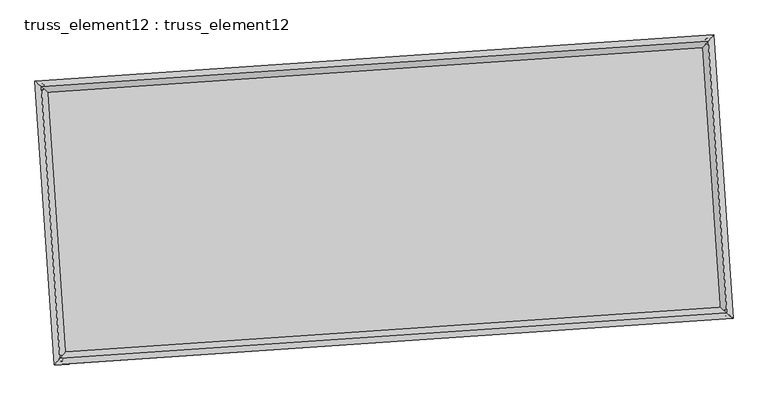
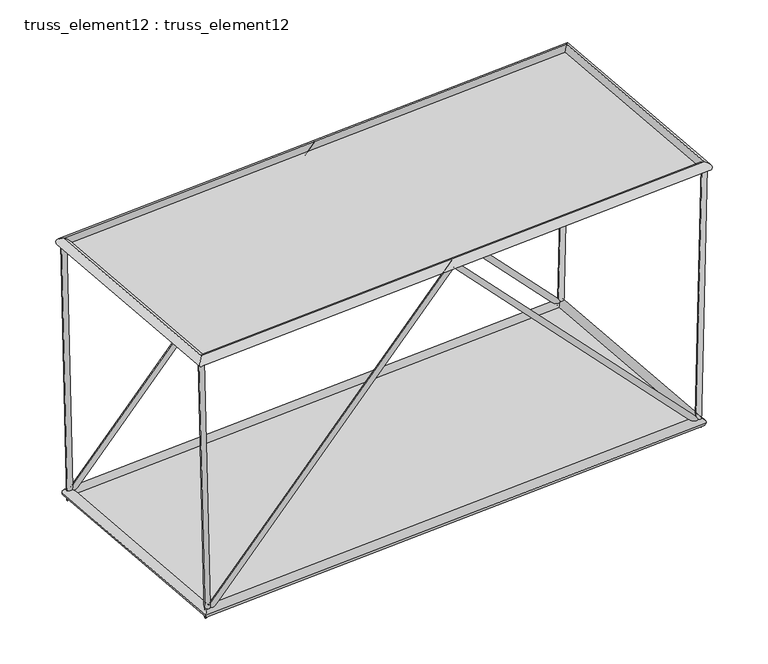
"""IFC4 building model written with IfcOpenShell, lengths in millimetres: plate geometry, truss_element12 : truss_element12."""

from ifc_helpers import new_model, si_unit, frame, origin, origin_with_axes, place, context, project, spatial, polyline, circle_curve, ellipse_curve, outline, extrude, source, transform, mapped, element, save
from ifc_brep_helpers import plane_surface, cylinder_surface, advanced_brep


def truss_element12_truss_element12_13b70bee(model_context):
    return source(origin(), model_context, "Body", "SolidModel", [
        advanced_brep(
        [(-3781.3878429, 2268.2839414, 4999.8023514), (-3880.4640895, 2254.9245561, 4997.4733651), (-3667.7523744, 2276.0323121, 121.2466732), (-3761.2345085, 2263.054368, -121.2466732), (1063.5274158, 2598.6402957, 5070.7560552), (1063.9784835, 2592.0672996, 4926.528566), (5795.1821195, 2921.2738432, 121.2492756), (5889.5788575, 2921.1066453, -121.2492756), (5908.4454526, 2928.9968394, 4999.8074441), (6008.4182784, 2929.2098536, 4997.4860818)],
        [
            (0, 1, circle_curve(frame((-3830.9259662, 2261.6042488, 4998.6378583), z_axis=(-0.02328650495741506, -0.0015878182527536, 0.9997275716514298), x_axis=(-0.13359443840271754, 0.9910348940631258, -0.001537783193974795)), 50.0)),
            (1, 0, circle_curve(frame((-3830.9259662, 2261.6042488, 4998.6378583), z_axis=(-0.02328650495741506, -0.0015878182527536, 0.9997275716514298), x_axis=(-0.13359443840271754, 0.9910348940631258, -0.001537783193974795)), 50.0)),
            (0, 2),
            (2, 3, ellipse_curve(frame((-3714.4934414, 2269.54334, 0.0), z_axis=(-0.9300456480783869, -0.06341627730797174, 0.36193019805323257), x_axis=(0.36109174913580183, 0.024621473735326325, 0.9322051982997884)), 130.347573, 50.0)),
            (3, 1),
            (3, 2, ellipse_curve(frame((-3714.4934414, 2269.54334, 0.0), z_axis=(-0.9300456480783869, -0.06341627730797174, 0.36193019805323257), x_axis=(0.36109174913580183, 0.024621473735326325, 0.9322051982997884)), 130.347573, 50.0)),
            (2, 4),
            (4, 5, ellipse_curve(frame((1063.7529497, 2595.3537976, 4998.6423106), z_axis=(-0.9976833958768767, -0.06802823821520047, -1.992283297939691e-05), x_axis=(1.9876679666230083e-05, 1.3553152281842393e-06, -0.9999999998015403)), 72.2707708, 50.0)),
            (5, 3),
            (5, 4, ellipse_curve(frame((1063.7529497, 2595.3537976, 4998.6423106), z_axis=(-0.9976833958768767, -0.06802823821520047, -1.992283297939691e-05), x_axis=(1.9876679666230083e-05, 1.3553152281842393e-06, -0.9999999998015403)), 72.2707708, 50.0)),
            (4, 6),
            (6, 7, ellipse_curve(frame((5842.3804885, 2921.1902443, 0.0), z_axis=(-0.9300246539008387, -0.06341484579481112, -0.3619843925771465), x_axis=(-0.3611458181124689, -0.024625160493309917, 0.9321841553741161)), 130.3533132, 50.0)),
            (7, 5),
            (7, 6, ellipse_curve(frame((5842.3804885, 2921.1902443, 0.0), z_axis=(-0.9300246539008387, -0.06341484579481112, -0.3619843925771465), x_axis=(-0.3611458181124689, -0.024625160493309917, 0.9321841553741161)), 130.3533132, 50.0)),
            (8, 9, circle_curve(frame((5958.4318655, 2929.1033465, 4998.6467629), z_axis=(0.023210275405573154, 0.0015826204493890937, 0.9997293525890448), x_axis=(-0.0021663046918160016, 0.9999964788957632, -0.0015327491829060865)), 50.0)),
            (9, 8, circle_curve(frame((5958.4318655, 2929.1033465, 4998.6467629), z_axis=(0.023210275405573154, 0.0015826204493890937, 0.9997293525890448), x_axis=(-0.0021663046918160016, 0.9999964788957632, -0.0015327491829060865)), 50.0)),
            (6, 8),
            (9, 7),
        ],
        [
            plane_surface(frame((-3830.9259662, 2311.6041857, 4998.7172707), z_axis=(-0.023286504957416205, -0.0015878182527521672, 0.9997275716514298), x_axis=(0.9997288325775486, -3.698476667768344e-05, 0.023286475586889552))),
            cylinder_surface(frame((-3830.9259662, 2261.6042488, 4998.6378583), z_axis=(-0.02328650495741506, -0.0015878182527536, 0.9997275716514298), x_axis=(-0.13359443840271754, 0.9910348940631258, -0.001537783193974795)), 50.0),
            cylinder_surface(frame((-3714.4934414, 2269.54334, 0.0), z_axis=(-0.6902255509886958, -0.047063856528962014, -0.7220621040956053), x_axis=(-0.02041790482368491, 0.9987519716635986, -0.045580788285038025)), 50.0),
            cylinder_surface(frame((1063.7529497, 2595.3537976, 4998.6423106), z_axis=(-0.690254254835047, -0.04706581373513127, 0.7220345371653382), x_axis=(-0.11534114330815694, 0.9922795168683531, -0.045582683816059205)), 50.0),
            plane_surface(frame((5958.4318655, 2879.1034091, 4998.7259153), z_axis=(0.023210275405573518, 0.0015826204493892728, 0.9997293525890449), x_axis=(0.9997306052710389, -3.674295485112107e-05, -0.023210246322644654))),
            cylinder_surface(frame((5842.3804885, 2921.1902443, 0.0), z_axis=(-0.023210275405573154, -0.0015826204493890937, -0.9997293525890448), x_axis=(-0.0021663046918160016, 0.9999964788957632, -0.0015327491829060865)), 50.0),
        ],
        [
            (0, [[1, 2]]),
            (1, [[-1, 3, 4, 5]]),
            (1, [[-2, -5, 6, -3]]),
            (2, [[-4, 7, 8, 9]]),
            (2, [[-6, -9, 10, -7]]),
            (3, [[-8, 11, 12, 13]]),
            (3, [[-10, -13, 14, -11]]),
            (4, [[15, 16]]),
            (5, [[-12, 17, -16, 18]]),
            (5, [[-14, -18, -15, -17]]),
        ],
    ),
        advanced_brep(
        [(-3509.27489, -1722.4496429, 4999.8023514), (-3608.3511366, -1735.8090282, 4997.4733651), (-3395.6394215, -1714.7012722, 121.2466732), (-3489.1215555, -1727.6792163, -121.2466732), (1335.6403687, -1392.0932886, 5070.7560552), (1336.0914364, -1398.6662847, 4926.528566), (6067.2950724, -1069.4597411, 121.2492756), (6161.6918104, -1069.626939, -121.2492756), (6180.5584055, -1061.7367449, 4999.8074441), (6280.5312314, -1061.5237307, 4997.4860818)],
        [
            (0, 1, circle_curve(frame((-3558.8130133, -1729.1293355, 4998.6378583), z_axis=(-0.023286504957415285, -0.0015878182527535897, 0.9997275716514298), x_axis=(-0.13359443840271787, 0.9910348940631256, -0.0015377831939748436)), 50.0)),
            (1, 0, circle_curve(frame((-3558.8130133, -1729.1293355, 4998.6378583), z_axis=(-0.023286504957415285, -0.0015878182527535897, 0.9997275716514298), x_axis=(-0.13359443840271787, 0.9910348940631256, -0.0015377831939748436)), 50.0)),
            (0, 2),
            (2, 3, ellipse_curve(frame((-3442.3804885, -1721.1902443, 0.0), z_axis=(-0.9300456480783867, -0.06341627730797184, 0.3619301980532322), x_axis=(0.3610917491358014, 0.024621473735326367, 0.9322051982997887)), 130.347573, 50.0)),
            (3, 1),
            (3, 2, ellipse_curve(frame((-3442.3804885, -1721.1902443, 0.0), z_axis=(-0.9300456480783867, -0.06341627730797184, 0.3619301980532322), x_axis=(0.3610917491358014, 0.024621473735326367, 0.9322051982997887)), 130.347573, 50.0)),
            (2, 4),
            (4, 5, ellipse_curve(frame((1335.8659026, -1395.3797867, 4998.6423106), z_axis=(-0.9976833958768767, -0.06802823821520053, -1.9922832979958566e-05), x_axis=(1.9876679666998888e-05, 1.3553152281361895e-06, -0.9999999998015403)), 72.2707708, 50.0)),
            (5, 3),
            (5, 4, ellipse_curve(frame((1335.8659026, -1395.3797867, 4998.6423106), z_axis=(-0.9976833958768767, -0.06802823821520053, -1.9922832979958566e-05), x_axis=(1.9876679666998888e-05, 1.3553152281361895e-06, -0.9999999998015403)), 72.2707708, 50.0)),
            (4, 6),
            (6, 7, ellipse_curve(frame((6114.4934414, -1069.54334, 0.0), z_axis=(-0.9300246539008382, -0.06341484579481105, -0.3619843925771475), x_axis=(-0.3611458181124699, -0.02462516049330997, 0.9321841553741157)), 130.3533132, 50.0)),
            (7, 5),
            (7, 6, ellipse_curve(frame((6114.4934414, -1069.54334, 0.0), z_axis=(-0.9300246539008382, -0.06341484579481105, -0.3619843925771475), x_axis=(-0.3611458181124699, -0.02462516049330997, 0.9321841553741157)), 130.3533132, 50.0)),
            (8, 9, circle_curve(frame((6230.5448184, -1061.6302378, 4998.6467629), z_axis=(0.023210275405571995, 0.0015826204493890016, 0.9997293525890449), x_axis=(-0.002166304691815724, 0.9999964788957632, -0.001532749182906003)), 50.0)),
            (9, 8, circle_curve(frame((6230.5448184, -1061.6302378, 4998.6467629), z_axis=(0.023210275405571995, 0.0015826204493890016, 0.9997293525890449), x_axis=(-0.002166304691815724, 0.9999964788957632, -0.001532749182906003)), 50.0)),
            (6, 8),
            (9, 7),
        ],
        [
            plane_surface(frame((-3558.8130133, -1679.1293986, 4998.7172707), z_axis=(-0.023286504957416205, -0.0015878182527521672, 0.9997275716514298), x_axis=(0.9997288325775486, -3.698476667768344e-05, 0.023286475586889552))),
            cylinder_surface(frame((-3558.8130133, -1729.1293355, 4998.6378583), z_axis=(-0.023286504957415282, -0.0015878182527535893, 0.9997275716514296), x_axis=(-0.13359443840271787, 0.9910348940631256, -0.0015377831939748436)), 50.0),
            cylinder_surface(frame((-3442.3804885, -1721.1902443, 0.0), z_axis=(-0.6902255509886953, -0.0470638565289621, -0.7220621040956057), x_axis=(-0.020417904823684878, 0.9987519716635985, -0.04558078828503815)), 50.0),
            cylinder_surface(frame((1335.8659026, -1395.3797867, 4998.6423106), z_axis=(-0.6902542548350474, -0.04706581373513127, 0.7220345371653377), x_axis=(-0.11534114330815701, 0.9922795168683533, -0.04558268381605939)), 50.0),
            plane_surface(frame((6230.5448184, -1111.6301752, 4998.7259153), z_axis=(0.023210275405573518, 0.0015826204493892728, 0.9997293525890449), x_axis=(0.9997306052710389, -3.674295485112107e-05, -0.023210246322644654))),
            cylinder_surface(frame((6114.4934414, -1069.54334, 0.0), z_axis=(-0.02321027540557199, -0.0015826204493890011, -0.9997293525890447), x_axis=(-0.002166304691815724, 0.9999964788957632, -0.001532749182906003)), 50.0),
        ],
        [
            (0, [[1, 2]]),
            (1, [[-1, 3, 4, 5]]),
            (1, [[-2, -5, 6, -3]]),
            (2, [[-4, 7, 8, 9]]),
            (2, [[-6, -9, 10, -7]]),
            (3, [[-8, 11, 12, 13]]),
            (3, [[-10, -13, 14, -11]]),
            (4, [[15, 16]]),
            (5, [[-12, 17, -16, 18]]),
            (5, [[-14, -18, -15, -17]]),
        ],
    ),
        advanced_brep(
        [(-3558.810702, -1729.1267739, 4908.6378583), (-3558.8153245, -1729.1318972, 5088.6378582), (-3830.9286038, 2261.606473, 5088.6378582), (-3830.9233286, 2261.6020246, 4908.6378583), (5958.4340138, 2929.105897, 5088.6467629), (5958.4297173, 2929.100796, 4908.646763), (6230.5472931, -1061.6324731, 5088.6467629), (6230.5423438, -1061.6280025, 4908.646763)],
        [
            (0, 1, ellipse_curve(frame((-3558.8130133, -1729.1293355, 4998.6378583), z_axis=(-0.7535719234051663, 0.6573654662781019, -6.417150933687318e-07), x_axis=(-0.6573654662777916, -0.753571923405437, -6.417150933687713e-07)), 127.2792206, 90.0)),
            (1, 2),
            (2, 3, ellipse_curve(frame((-3830.9259662, 2261.6042488, 4998.6378583), z_axis=(-0.6573654662777915, -0.7535719234054372, -6.417150933688095e-07), x_axis=(0.7535719234051665, -0.6573654662781016, 6.417150933687701e-07)), 127.2792206, 90.0)),
            (3, 0),
            (1, 0, ellipse_curve(frame((-3558.8130133, -1729.1293355, 4998.6378583), z_axis=(-0.7535719234051663, 0.6573654662781019, -6.417150933687318e-07), x_axis=(-0.6573654662777916, -0.753571923405437, -6.417150933687713e-07)), 127.2792206, 90.0)),
            (3, 2, ellipse_curve(frame((-3830.9259662, 2261.6042488, 4998.6378583), z_axis=(-0.6573654662777915, -0.7535719234054372, -6.417150933688095e-07), x_axis=(0.7535719234051665, -0.6573654662781016, 6.417150933687701e-07)), 127.2792206, 90.0)),
            (2, 4),
            (4, 5, ellipse_curve(frame((5958.4318655, 2929.1033465, 4998.6467629), z_axis=(-0.7535719234051664, 0.6573654662781019, -6.41715093368808e-07), x_axis=(-0.6573654662777914, -0.7535719234054371, -6.417150933687716e-07)), 127.2792206, 90.0)),
            (5, 3),
            (5, 4, ellipse_curve(frame((5958.4318655, 2929.1033465, 4998.6467629), z_axis=(-0.7535719234051664, 0.6573654662781019, -6.41715093368808e-07), x_axis=(-0.6573654662777914, -0.7535719234054371, -6.417150933687716e-07)), 127.2792206, 90.0)),
            (4, 6),
            (6, 7, ellipse_curve(frame((6230.5448184, -1061.6302378, 4998.6467629), z_axis=(0.6573654662777916, 0.753571923405437, 6.417150933687335e-07), x_axis=(-0.7535719234051662, 0.657365466278102, -6.417150933687697e-07)), 127.2792206, 90.0)),
            (7, 5),
            (7, 6, ellipse_curve(frame((6230.5448184, -1061.6302378, 4998.6467629), z_axis=(0.6573654662777916, 0.753571923405437, 6.417150933687335e-07), x_axis=(-0.7535719234051662, 0.657365466278102, -6.417150933687697e-07)), 127.2792206, 90.0)),
            (6, 1),
            (0, 7),
        ],
        [
            cylinder_surface(frame((-3558.8130133, -1729.1293355, 4998.6378583), z_axis=(0.06802823822869986, -0.9976833960748767, 0.0), x_axis=(-0.997683395696052, -0.06802823820286925, -2.7557367220821507e-05)), 90.0),
            cylinder_surface(frame((-3830.9259662, 2261.6042488, 4998.6378583), z_axis=(-0.9976833960744659, -0.06802823822867164, -9.075221882216596e-07), x_axis=(-0.06802823818041304, 0.9976833957222375, -2.6649845032922138e-05)), 90.0),
            cylinder_surface(frame((5958.4318655, 2929.1033465, 4998.6467629), z_axis=(-0.06802823822869951, 0.9976833960748768, 0.0), x_axis=(0.9976833957443108, 0.06802823820615947, -2.5742322845022792e-05)), 90.0),
            cylinder_surface(frame((6230.5448184, -1061.6302378, 4998.6467629), z_axis=(0.997683396074466, 0.06802823822867146, 9.075221882216056e-07), x_axis=(0.06802823822867146, -0.997683395718947, -2.6649845032922155e-05)), 90.0),
        ],
        [
            (0, [[1, 2, 3, 4]]),
            (0, [[5, -4, 6, -2]]),
            (1, [[-3, 7, 8, 9]]),
            (1, [[-6, -9, 10, -7]]),
            (2, [[-8, 11, 12, 13]]),
            (2, [[-10, -13, 14, -11]]),
            (3, [[-12, 15, -1, 16]]),
            (3, [[-14, -16, -5, -15]]),
        ],
    ),
        advanced_brep(
        [(-3358.7115243, -1625.2761972, 0.0), (-3526.0494527, -1817.1042913, 0.0), (-3810.4074885, 2353.2123043, 0.0), (-3618.5793943, 2185.8743758, 0.0), (5926.0494527, 3017.1042913, 0.0), (5758.7115243, 2825.2761972, 0.0), (6210.4074885, -1153.2123043, 0.0), (6018.5793943, -985.8743758, 0.0)],
        [
            (0, 1, ellipse_curve(frame((-3442.3804885, -1721.1902443, 0.0), z_axis=(-0.7535719234054579, 0.6573654662780808, 0.0), x_axis=(-0.6573654662780808, -0.753571923405458, 0.0)), 127.2792206, 90.0)),
            (1, 2),
            (2, 3, ellipse_curve(frame((-3714.4934414, 2269.54334, 0.0), z_axis=(-0.6573654662780807, -0.7535719234054581, 0.0), x_axis=(0.7535719234054581, -0.6573654662780806, 0.0)), 127.2792206, 90.0)),
            (3, 0),
            (1, 0, ellipse_curve(frame((-3442.3804885, -1721.1902443, 0.0), z_axis=(-0.7535719234054579, 0.6573654662780808, 0.0), x_axis=(-0.6573654662780808, -0.753571923405458, 0.0)), 127.2792206, 90.0)),
            (3, 2, ellipse_curve(frame((-3714.4934414, 2269.54334, 0.0), z_axis=(-0.6573654662780807, -0.7535719234054581, 0.0), x_axis=(0.7535719234054581, -0.6573654662780806, 0.0)), 127.2792206, 90.0)),
            (2, 4),
            (4, 5, ellipse_curve(frame((5842.3804885, 2921.1902443, 0.0), z_axis=(-0.7535719234054578, 0.657365466278081, 0.0), x_axis=(-0.657365466278081, -0.7535719234054578, 0.0)), 127.2792206, 90.0)),
            (5, 3),
            (5, 4, ellipse_curve(frame((5842.3804885, 2921.1902443, 0.0), z_axis=(-0.7535719234054578, 0.657365466278081, 0.0), x_axis=(-0.657365466278081, -0.7535719234054578, 0.0)), 127.2792206, 90.0)),
            (4, 6),
            (6, 7, ellipse_curve(frame((6114.4934414, -1069.54334, 0.0), z_axis=(0.6573654662780811, 0.7535719234054576, 0.0), x_axis=(-0.7535719234054576, 0.6573654662780812, 0.0)), 127.2792206, 90.0)),
            (7, 5),
            (7, 6, ellipse_curve(frame((6114.4934414, -1069.54334, 0.0), z_axis=(0.6573654662780811, 0.7535719234054576, 0.0), x_axis=(-0.7535719234054576, 0.6573654662780812, 0.0)), 127.2792206, 90.0)),
            (6, 1),
            (0, 7),
        ],
        [
            cylinder_surface(frame((-3442.3804885, -1721.1902443, 0.0), z_axis=(0.06802823822870163, -0.9976833960748767, 0.0), x_axis=(-0.9976833960748767, -0.06802823822870163, 0.0)), 90.0),
            cylinder_surface(frame((-3714.4934414, 2269.54334, 0.0), z_axis=(-0.9976833960748767, -0.06802823822870106, 0.0), x_axis=(-0.06802823822870106, 0.9976833960748767, 0.0)), 90.0),
            cylinder_surface(frame((5842.3804885, 2921.1902443, 0.0), z_axis=(-0.06802823822870085, 0.9976833960748767, 0.0), x_axis=(0.9976833960748767, 0.06802823822870085, 0.0)), 90.0),
            cylinder_surface(frame((6114.4934414, -1069.54334, 0.0), z_axis=(0.9976833960748767, 0.06802823822870076, 0.0), x_axis=(0.06802823822870076, -0.9976833960748767, 0.0)), 90.0),
        ],
        [
            (0, [[1, 2, 3, 4]]),
            (0, [[5, -4, 6, -2]]),
            (1, [[-3, 7, 8, 9]]),
            (1, [[-6, -9, 10, -7]]),
            (2, [[-8, 11, 12, 13]]),
            (2, [[-10, -13, 14, -11]]),
            (3, [[-12, 15, -1, 16]]),
            (3, [[-14, -16, -5, -15]]),
        ],
    ),
        extrude(outline(polyline([(-3442.3804885, -1721.1902443), (-3714.4934414, 2269.54334), (5842.3804885, 2921.1902443), (6114.4934414, -1069.54334), (-3442.3804885, -1721.1902443)])), origin_with_axes(), (0.0, 0.0, 1.0), 20.0),
        extrude(outline(polyline([(-2000.0, 4906.0442773), (2000.0, 4906.0442773), (2000.0, -4906.0442773), (-2000.0, -4906.0442773), (-2000.0, 4906.0442773)])), frame((1199.8094261, 599.9870055, 4998.6423106), z_axis=(-9.054198187582621e-07, -6.173713561817364e-08, 0.9999999999995883), x_axis=(-0.06802823822870142, 0.9976833960748767, 0.0)), (0.0, 0.0, 1.0), 20.0),
    ])


if __name__ == "__main__":
    model = new_model("IFC4")
    model_context = context("Model", 3, world=origin())
    ifc_project = project(units=[si_unit("LENGTHUNIT", "METRE", prefix="MILLI")], contexts=[model_context])
    site = spatial("IfcSite", under=ifc_project)
    building = spatial("IfcBuilding", under=site)
    placement = place(None, origin())
    truss_element12_truss_element12_shape = truss_element12_truss_element12_13b70bee(model_context)
    element("IfcPlate", 1, ObjectType="truss_element12 : truss_element12", at=placement, inside=building, context=model_context, shape_type="MappedRepresentation", body=[
        mapped(truss_element12_truss_element12_shape, transform((0.0, 0.0, 0.0), x_axis=(1.0, 0.0, 0.0), y_axis=(0.0, 1.0, 0.0), z_axis=(0.0, 0.0, 1.0))),
    ])
    save(model, "model.ifc")

# Revit data of these elements
# Type "truss_element12 : truss_element12"
#   steellbar1 = 90 mm
#   steelbar2 = 50 mm
#   offset1 = 5000 mm
#   M = Default Roof
# Element 1 (IfcPlate, "truss_element12 : truss_element12")
#   Materials on its faces: "Default Roof"
# Materials
#   "Default Roof": class "Miscellaneous", colour RGB 0 127 0, transparency 0, Comments = "Rendering appearance not upgraded Rendering appearance not upgraded ", Cost = 0
